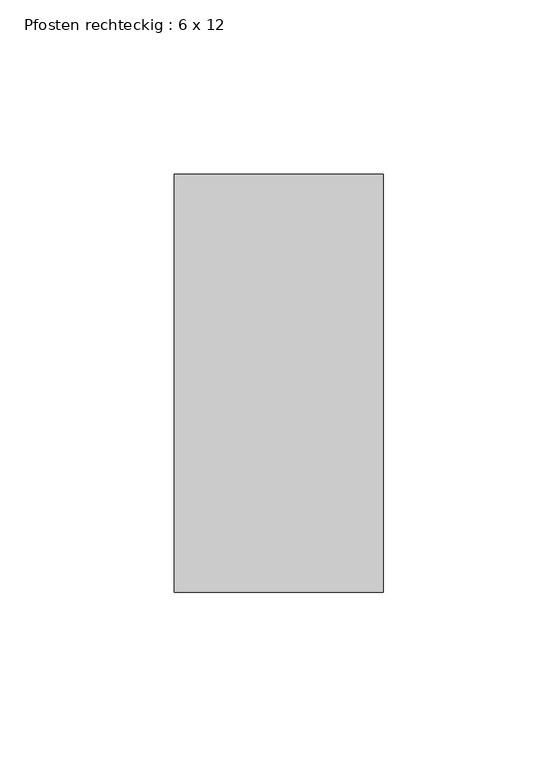
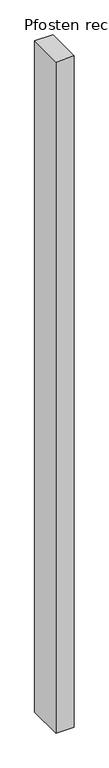
"""IFC4 building model written with IfcOpenShell, lengths in millimetres: member geometry, Pfosten rechteckig : 6 x 12."""

from ifc_helpers import new_model, si_unit, frame, origin, place, context, project, spatial, polyline, outline, extrude, source, transform, mapped, element, save


def pfosten_rechteckig_6_x_12_8a56a971(model_context):
    return source(origin(), model_context, "Body", "SweptSolid", [
        extrude(outline(polyline([(30.0, 60.0), (30.0, -60.0), (-30.0, -60.0), (-30.0, 60.0), (30.0, 60.0)])), frame((0.0, 0.0, -2320.0), z_axis=(0.0, 0.0, 1.0), x_axis=(1.0, 0.0, 0.0)), (0.0, 0.0, 1.0), 2320.0),
    ])


if __name__ == "__main__":
    model = new_model("IFC4")
    model_context = context("Model", 3, world=origin())
    ifc_project = project(units=[si_unit("LENGTHUNIT", "METRE", prefix="MILLI")], contexts=[model_context])
    site = spatial("IfcSite", under=ifc_project)
    building = spatial("IfcBuilding", under=site)
    placement = place(None, origin())
    pfosten_rechteckig_6_x_12_shape = pfosten_rechteckig_6_x_12_8a56a971(model_context)
    element("IfcMember", 1, ObjectType="Pfosten rechteckig : 6 x 12", at=placement, inside=building, context=model_context, shape_type="MappedRepresentation", body=[
        mapped(pfosten_rechteckig_6_x_12_shape, transform((0.0, 0.0, 0.0), x_axis=(1.0, 0.0, 0.0), y_axis=(0.0, 1.0, 0.0), z_axis=(0.0, 0.0, 1.0))),
    ])
    save(model, "model.ifc")

# Revit data of these elements
# Type "Pfosten rechteckig : 6 x 12"
#   built-in parameter 1007304 = 0.393701 (stored number, unit not read)
#   built-in parameter 1007301 = 0.0984252 (stored number, unit not read)
#   built-in parameter 1007300 = 0.0984252 (stored number, unit not read)
# Element 1 (IfcMember, "Pfosten rechteckig : 6 x 12")
#   Materials on its faces: "Metall - verzinkt"
# Materials
#   "Metall - verzinkt": class "Allgemeines", colour RGB 200 200 200, transparency 0, Cost = 0
